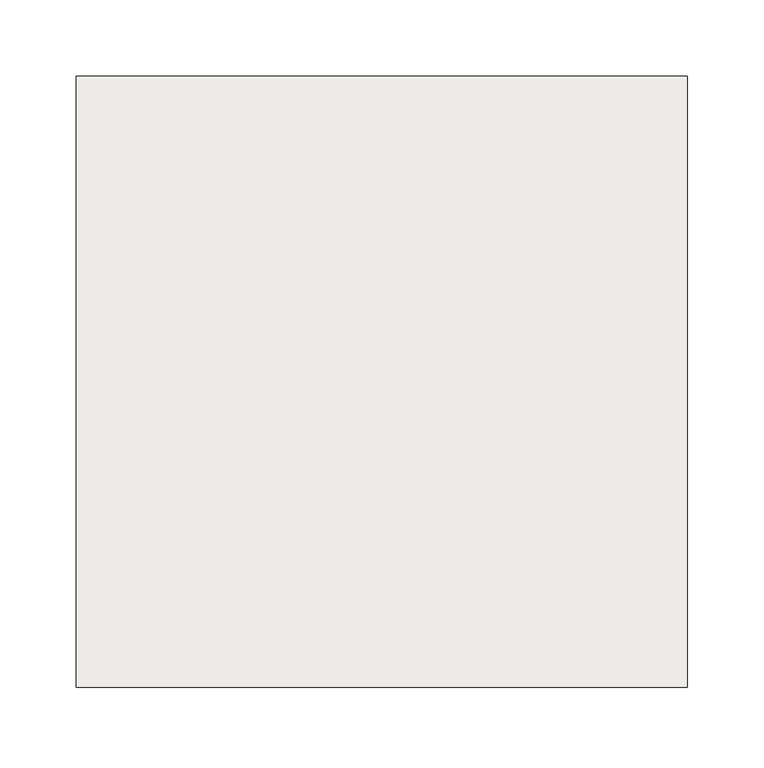
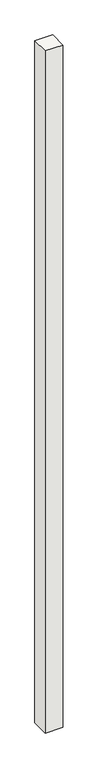
"""IFC4 building model written with IfcOpenShell, lengths in millimetres: footing geometry, NLRS_17_SFO_TLB_funderingspaal geheid beton prefab-AV-MMBPC_gen_rsf : heipaal beton prefab_gen__bxh 400x400."""

from ifc_helpers import new_model, si_unit, frame, origin, place, context, project, spatial, polyline, outline, extrude, source, transform, mapped, element, save


def footing_d279473c(model_context):
    return source(origin(), model_context, "Body", "SweptSolid", [
        extrude(outline(polyline([(200.0, -200.0), (-200.0, -200.0), (-200.0, 200.0), (200.0, 200.0), (200.0, -200.0)])), frame((0.0, 0.0, -20000.0), z_axis=(0.0, 0.0, 1.0), x_axis=(1.0, 0.0, 0.0)), (0.0, 0.0, 1.0), 16250.0),
    ])


if __name__ == "__main__":
    model = new_model("IFC4")
    model_context = context("Model", 3, world=origin())
    ifc_project = project(units=[si_unit("LENGTHUNIT", "METRE", prefix="MILLI")], contexts=[model_context])
    site = spatial("IfcSite", under=ifc_project)
    building = spatial("IfcBuilding", under=site)
    placement = place(None, origin())
    footing_shape = footing_d279473c(model_context)
    element("IfcFooting", 1, ObjectType="NLRS_17_SFO_TLB_funderingspaal geheid beton prefab-AV-MMBPC_gen_rsf : heipaal beton prefab_gen__bxh 400x400", at=placement, inside=building, context=model_context, shape_type="MappedRepresentation", body=[
        mapped(footing_shape, transform((0.0, 0.0, 0.0), x_axis=(1.0, 0.0, 0.0), y_axis=(0.0, 1.0, 0.0), z_axis=(0.0, 0.0, 1.0))),
    ])
    save(model, "model.ifc")

# Revit data of these elements
# Type "NLRS_17_SFO_TLB_funderingspaal geheid beton prefab-AV-MMBPC_gen_rsf : heipaal beton prefab_gen__bxh 400x400"
#   IfcExportAs = "IfcPile"
#   Type Comments = "prefab heipaal 400x400"
#   Model = " "
#   Manufacturer = " "
#   Description = "prefab heipaal 400x400"
#   Assembly Code = "17.21"
#   Width = 400 mm
#   Slanted Angle [instance default] = 0.00°
#   NLRS_S_draagvermogen_trek [instance default] = 0.00 kN
#   NLRS_S_draagvermogen_druk [instance default] = 0.00 kN
#   NLRS_C_lengte [instance default] = 1660 mm
#   NLRS_C_hoogte = 400 mm
#   NLRS_C_breedte = 400 mm
#   Height [instance default] = 1660 mm
#   Length [instance default] = 1660 mm
#   Angle [instance default] = 0.00°
#   Slanted [instance default] = 0
#   Structural Material = NLRS_f2_beton prefab_gen_rsf
#   Keynote = ""
# Element 1 (IfcFooting, "NLRS_17_SFO_TLB_funderingspaal geheid beton prefab-AV-MMBPC_gen_rsf : heipaal beton prefab_gen__bxh 400x400")
#   NLRS_C_lengte = 16250 mm
#   Height = 16250 mm
#   Length = 16250 mm
#   Materials on its faces: "NLRS_f2_beton prefab_gen_rsf"
# Materials
#   "NLRS_f2_beton prefab_gen_rsf": class "F - Niet gebakken kunststeen", colour RGB 129 133 118, transparency 0, Keynote = "f2", Manufacturer = "Revit Standards Foundation", URL = "www.revitstandards.org", Description = "beton prefab", Cost = 0
